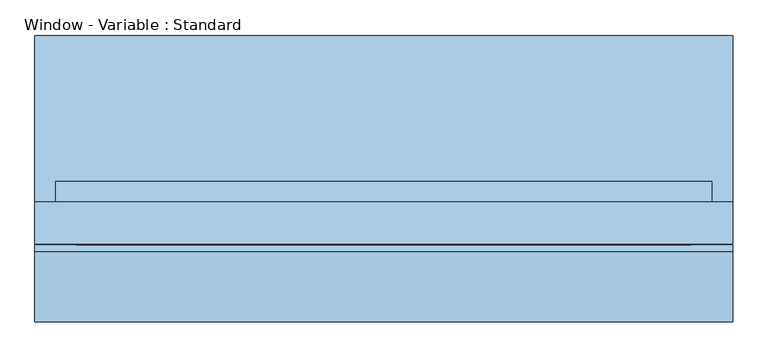
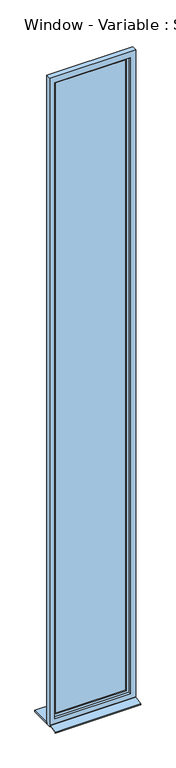
"""IFC4 building model written with IfcOpenShell, lengths in millimetres: window geometry, Window - Variable : Standard."""

from ifc_helpers import new_model, si_unit, frame, origin, place, context, project, spatial, polyline, outline, extrude, faceted_brep, source, transform, mapped, element, save


def window_variable_standard_e4ea84a9(model_context):
    return source(origin(), model_context, "Body", "SolidModel", [
        extrude(outline(polyline([(9000.0, 500.0), (9000.0, -500.0), (1000.0, -500.0), (1000.0, 500.0), (9000.0, 500.0)]), holes=[polyline([(8920.0, 440.0), (1080.0, 440.0), (1080.0, -440.0), (8920.0, -440.0), (8920.0, 440.0)])]), frame((0.0, -95.0, 0.0), z_axis=(0.0, 1.0, 0.0), x_axis=(0.0, 0.0, 1.0)), (0.0, 0.0, 1.0), 60.0),
        faceted_brep([(470.0, -35.0, 8950.0), (470.0, -35.0, 1050.0), (470.0, -5.0, 1050.0), (470.0, -5.0, 8950.0), (-470.0, -5.0, 1050.0), (-470.0, -5.0, 8950.0), (410.0, -5.0, 1110.0), (410.0, -5.0, 8890.0), (-410.0, -5.0, 8890.0), (-410.0, -5.0, 1110.0), (-470.0, -35.0, 1050.0), (-470.0, -35.0, 8950.0), (440.0, -35.0, 8920.0), (440.0, -35.0, 1080.0), (-440.0, -35.0, 1080.0), (-440.0, -35.0, 8920.0), (440.0, -65.0, 8920.0), (440.0, -65.0, 1080.0), (-440.0, -65.0, 1080.0), (-440.0, -65.0, 8920.0), (410.0, -65.0, 8890.0), (410.0, -65.0, 1110.0), (-410.0, -65.0, 1110.0), (-410.0, -65.0, 8890.0)], [[[0, 1, 2, 3]], [[3, 2, 4, 5], [6, 7, 8, 9]], [[1, 10, 4, 2]], [[1, 0, 11, 10], [12, 13, 14, 15]], [[16, 17, 13, 12]], [[17, 18, 14, 13]], [[17, 16, 19, 18], [20, 21, 22, 23]], [[7, 6, 21, 20]], [[6, 9, 22, 21]], [[10, 11, 5, 4]], [[18, 19, 15, 14]], [[9, 8, 23, 22]], [[11, 0, 3, 5]], [[19, 16, 12, 15]], [[8, 7, 20, 23]]]),
        extrude(outline(polyline([(-500.0, 205.0), (500.0, 205.0), (500.0, -35.0), (-500.0, -35.0), (-500.0, 205.0)])), frame((0.0, 0.0, 1005.0), z_axis=(0.0, 0.0, 1.0), x_axis=(1.0, 0.0, 0.0)), (0.0, 0.0, 1.0), 15.0),
        extrude(outline(polyline([(-105.0221543, 1020.0), (-95.0, 1020.0), (-95.0, 1018.0), (-104.8240723, 1018.0), (-203.0, 998.3604634), (-203.0, 990.0), (-205.0, 990.0), (-205.0, 1000.0), (-105.0221543, 1020.0)])), frame((-500.0, 0.0, 0.0), z_axis=(1.0, 0.0, 0.0), x_axis=(0.0, 1.0, 0.0)), (0.0, 0.0, 1.0), 1000.0),
        extrude(outline(polyline([(410.0, -20.0), (410.0, -50.0), (-410.0, -50.0), (-410.0, -20.0), (410.0, -20.0)])), frame((0.0, 0.0, 1110.0), z_axis=(0.0, 0.0, 1.0), x_axis=(1.0, 0.0, 0.0)), (0.0, 0.0, 1.0), 7780.0),
    ])


if __name__ == "__main__":
    model = new_model("IFC4")
    model_context = context("Model", 3, world=origin())
    ifc_project = project(units=[si_unit("LENGTHUNIT", "METRE", prefix="MILLI")], contexts=[model_context])
    site = spatial("IfcSite", under=ifc_project)
    building = spatial("IfcBuilding", under=site)
    placement = place(None, origin())
    window_variable_standard_shape = window_variable_standard_e4ea84a9(model_context)
    element("IfcWindow", 1, ObjectType="Window - Variable : Standard", at=placement, inside=building, context=model_context, shape_type="MappedRepresentation", body=[
        mapped(window_variable_standard_shape, transform((0.0, 0.0, 0.0), x_axis=(1.0, 0.0, 0.0), y_axis=(0.0, 1.0, 0.0), z_axis=(0.0, 0.0, 1.0))),
    ])
    save(model, "model.ifc")

# Revit data of these elements
# Type "Window - Variable : Standard"
#   Type Mark = "19"
#   Operation = "SinglePanel"
#   Keynote = "16.05.01"
#   Analytic Construction = "<None>"
#   Rough Width [instance default] = 1.010 m
#   Rough Height [instance default] = 1.010 m
#   Frame Depth = 0.060 m
#   Frame Height Bottom = 0.080 m
#   Frame Height Top = 0.080 m
#   Frame Width = 0.060 m
#   Height [instance default] = 1.010 m
#   Window Inset = 0.060 m
#   Window Width = 0.060 m
#   Instalation Depth [instance default] = 0.080 m
#   Width [instance default] = 1.010 m
#   Folding Wing [instance default] = no
#   Oppening Direction Vertical [instance default] = yes
#   Oppening Direction Visibility [instance default] = no
#   Casement [instance default] = yes
#   Frame [instance default] = none
#   Glas [instance default] = none
#   Window [instance default] = none
#   Windowsill Inside [instance default] = none
#   Windowsill Outside [instance default] = none
#   Wall Closure = (empty or 0)
#   Assembly Code = ""
# Element 1 (IfcWindow, "Window - Variable : Standard")
#   Rough Width = 1.000 m
#   Rough Height = 8.000 m
#   Height = 8.000 m
#   Width = 1.000 m
#   Materials on its faces: "Plastic - White", "Metal _ Aluminium", "Wood - Birch", "Glass"
# Materials
#   "Plastic - White": class "Kunststoff", colour RGB 249 249 249, transparency 0
#   "Metal _ Aluminium": class "Metall", colour RGB 247 247 247, transparency 0
#   "Wood - Birch": class "Holz", colour RGB 213 164 103, transparency 0
#   "Glass": class "Glass", colour RGB 0 128 192, transparency 0.9
